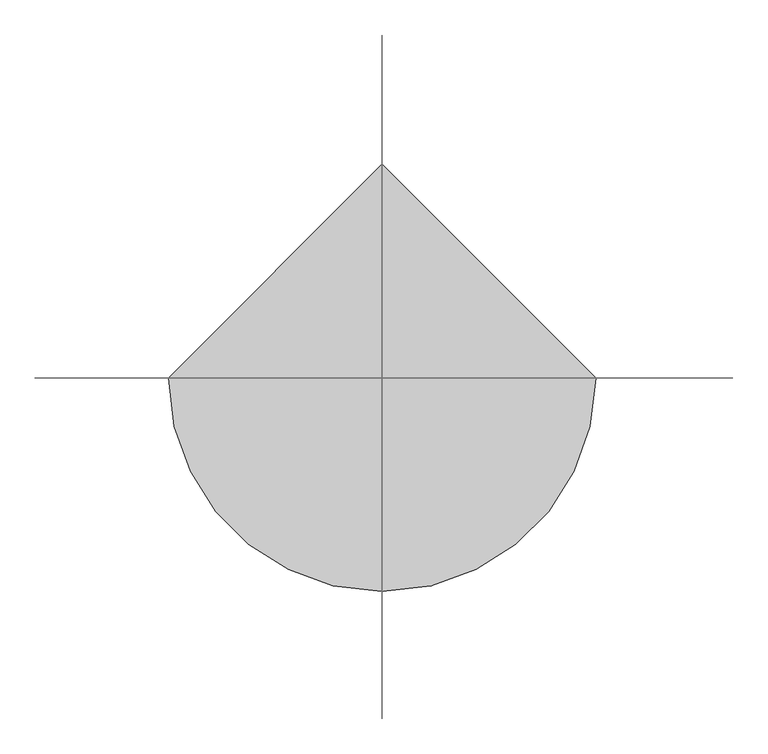
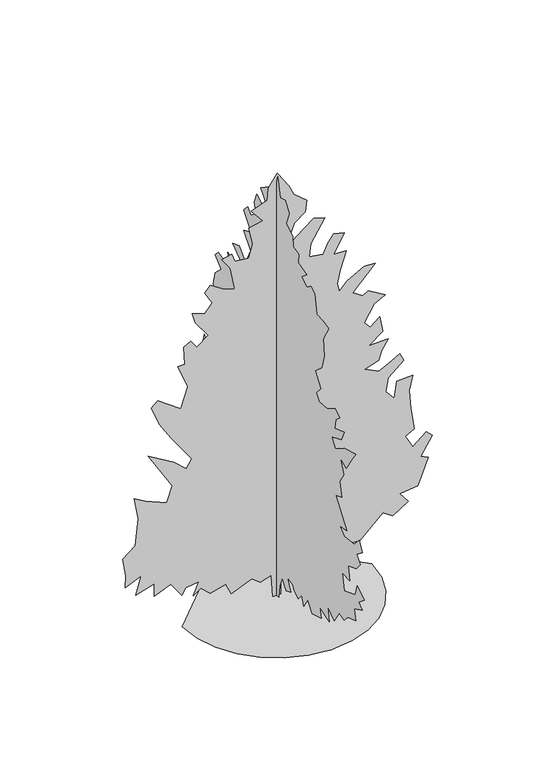
"""IFC4 building model written with IfcOpenShell, lengths in millimetres: proxy geometry, holly miniature 26078 : holly miniature 26078."""

import ifcopenshell
import ifcopenshell.guid

model = None  # the IFC model being written
_history = None  # IfcOwnerHistory: only IFC2X3 demands one
_inside = {}  # id of a spatial element -> (the spatial element, [elements in it])
_under = {}  # id of a project, library or spatial element -> (it, [spatial elements below it])
_declared = {}  # id of a project -> (the project, [libraries it declares])
_typed = {}  # id of a type object -> (the type object, [elements of that type])
_made_of = {}  # id of a material, layer set ... -> (it, [elements and type objects made of it])


def new_model(schema):
    """Start an empty IFC model of exactly this schema.

    Asked for "IFC4X3", IfcOpenShell would pick the latest addendum, in which some entities
    have other attributes; the version numbers below select the first issue.
    IFC2X3 requires an IfcOwnerHistory on every rooted entity: one is made here for all.
    """
    global model, _history
    if schema == "IFC4X3":
        model = ifcopenshell.file(schema_version=(4, 3, 0, 0))
    else:
        model = ifcopenshell.file(schema=schema)
    _inside.clear()
    _under.clear()
    _declared.clear()
    _typed.clear()
    _made_of.clear()
    _history = None
    if model.schema == "IFC2X3":
        org = make("IfcOrganization", Name="unknown")
        user = make(
            "IfcPersonAndOrganization",
            ThePerson=make("IfcPerson", FamilyName="unknown"),
            TheOrganization=org,
        )
        app = make(
            "IfcApplication",
            ApplicationDeveloper=org,
            Version="unknown",
            ApplicationFullName="unknown",
            ApplicationIdentifier="unknown",
        )
        _history = make(
            "IfcOwnerHistory",
            OwningUser=user,
            OwningApplication=app,
            ChangeAction="ADDED",
            CreationDate=0,
        )
    return model


def make(cls, **values):
    """One entity of the class cls with the attributes given. An attribute that is None is left unset."""
    return model.create_entity(
        cls, **{name: value for name, value in values.items() if value is not None}
    )


def rooted(cls, **values):
    """An entity with a GlobalId (a new one), such as an element, a storey or a relation."""
    return make(cls, GlobalId=ifcopenshell.guid.new(), OwnerHistory=_history, **values)


def si_unit(unit_type, name, prefix=None):
    """IfcSIUnit, for example si_unit("LENGTHUNIT", "METRE", prefix="MILLI")."""
    return make("IfcSIUnit", UnitType=unit_type, Prefix=prefix, Name=name)


def assignment(units):
    """IfcUnitAssignment: the units of a project."""
    return None if units is None else make("IfcUnitAssignment", Units=units)


def point(xyz):
    """IfcCartesianPoint."""
    return None if xyz is None else make("IfcCartesianPoint", Coordinates=xyz)


def direction(xyz):
    """IfcDirection."""
    return None if xyz is None else make("IfcDirection", DirectionRatios=xyz)


def frame(location, z_axis=None, x_axis=None):
    """IfcAxis2Placement3D, a coordinate frame: its origin and axes. An axis left out is left unset."""
    return make(
        "IfcAxis2Placement3D",
        Location=point(location),
        Axis=direction(z_axis),
        RefDirection=direction(x_axis),
    )


def origin():
    """The frame at (0, 0, 0) with its axes left unset."""
    return frame((0.0, 0.0, 0.0))


def place(relative_to, where):
    """IfcLocalPlacement: puts the frame where relative to a parent placement (None: the world)."""
    return make(
        "IfcLocalPlacement", PlacementRelTo=relative_to, RelativePlacement=where
    )


def context(
    kind, dimensions, precision=None, world=None, true_north=None, identifier=None
):
    """IfcGeometricRepresentationContext, for example the 3D "Model" context."""
    return make(
        "IfcGeometricRepresentationContext",
        ContextIdentifier=identifier,
        ContextType=kind,
        CoordinateSpaceDimension=dimensions,
        Precision=precision,
        WorldCoordinateSystem=world,
        TrueNorth=true_north,
    )


def project(units=None, contexts=None):
    """IfcProject with its units and contexts."""
    return rooted(
        "IfcProject",
        Name="project",
        RepresentationContexts=contexts,
        UnitsInContext=assignment(units),
    )


def spatial(cls, under=None, at=None, **own):
    """A site, building, storey or space (cls), placed at a placement, below another one or the project."""
    s = rooted(cls, ObjectPlacement=at, **own)
    if under is not None:
        _under.setdefault(under.id(), (under, []))[1].append(s)
    return s


def point_list(points):
    """IfcCartesianPointList2D or 3D."""
    cls = (
        "IfcCartesianPointList2D" if len(points[0]) == 2 else "IfcCartesianPointList3D"
    )
    return make(cls, CoordList=points)


def triangles(points, corners, closed=None, point_numbers=None):
    """IfcTriangulatedFaceSet: each triangle names its three corners, points numbered from 1."""
    return make(
        "IfcTriangulatedFaceSet",
        Coordinates=point_list(points),
        Closed=closed,
        CoordIndex=corners,
        PnIndex=point_numbers,
    )


def shape(context_of_items, identifier, shape_type, items):
    """IfcShapeRepresentation: the items that make up one representation, for example the "Body"."""
    return make(
        "IfcShapeRepresentation",
        ContextOfItems=context_of_items,
        RepresentationIdentifier=identifier,
        RepresentationType=shape_type,
        Items=items,
    )


def source(mapping_origin, context_of_items, identifier, shape_type, items):
    """IfcRepresentationMap: a shape defined once, which mapped items show again and again."""
    return make(
        "IfcRepresentationMap",
        MappingOrigin=mapping_origin,
        MappedRepresentation=shape(context_of_items, identifier, shape_type, items),
    )


def transform(
    local_origin,
    x_axis=None,
    y_axis=None,
    z_axis=None,
    scale=None,
    scale2=None,
    scale3=None,
    uniform=True,
):
    """IfcCartesianTransformationOperator3D, or its non-uniform kind. x_axis, y_axis, z_axis: its Axis1, 2, 3."""
    if uniform:
        return make(
            "IfcCartesianTransformationOperator3D",
            Axis1=direction(x_axis),
            Axis2=direction(y_axis),
            LocalOrigin=point(local_origin),
            Scale=scale,
            Axis3=direction(z_axis),
        )
    return make(
        "IfcCartesianTransformationOperator3DnonUniform",
        Axis1=direction(x_axis),
        Axis2=direction(y_axis),
        LocalOrigin=point(local_origin),
        Scale=scale,
        Axis3=direction(z_axis),
        Scale2=scale2,
        Scale3=scale3,
    )


def mapped(mapping_source, mapping_target):
    """IfcMappedItem: shows the shape of a source again, moved by a transform."""
    return make(
        "IfcMappedItem", MappingSource=mapping_source, MappingTarget=mapping_target
    )


def made_of(thing, what):
    """Note that an element or type object is made of a material, layer set ...; save() writes the relation."""
    if what is not None:
        _made_of.setdefault(what.id(), (what, []))[1].append(thing)
    return thing


def element(
    cls,
    number,
    at=None,
    inside=None,
    cuts=None,
    type_object=None,
    material=None,
    context=None,
    identifier="Body",
    shape_type=None,
    held_by="IfcProductDefinitionShape",
    body=None,
    shapes=None,
    **own,
):
    """One element of the class cls, such as IfcWall. Its Tag is "e" and its number.

    at: its placement. inside: the storey or other place that contains it. cuts: it is an
    opening in that element (IfcRelVoidsElement). A single representation is given by context,
    identifier, shape_type and body (its items); several are given by shapes. held_by: the class
    of the entity that holds the representations. save() writes the other relations.
    """
    e = rooted(cls, Tag="e%d" % number, ObjectPlacement=at, **own)
    if body is not None:
        shapes = [shape(context, identifier, shape_type, body)]
    if shapes is not None:
        e.Representation = make(held_by, Representations=shapes)
    if inside is not None:
        _inside.setdefault(inside.id(), (inside, []))[1].append(e)
    if cuts is not None:
        rooted(
            "IfcRelVoidsElement", RelatingBuildingElement=cuts, RelatedOpeningElement=e
        )
    if type_object is not None:
        _typed.setdefault(type_object.id(), (type_object, []))[1].append(e)
    return made_of(e, material)


def aggregate(whole, parts):
    """IfcRelAggregates: a whole, such as a stair, and the parts it consists of."""
    return rooted("IfcRelAggregates", RelatingObject=whole, RelatedObjects=parts)


def save(model, path):
    """Write the relations noted so far, then the file.

    IfcRelAggregates (storeys below a building ...), IfcRelContainedInSpatialStructure (elements
    in a storey), IfcRelDefinesByType, IfcRelAssociatesMaterial and IfcRelDeclares: one each for
    every whole, place, type object, material and project.
    """
    for whole, parts in _under.values():
        aggregate(whole, parts)
    for where, things in _inside.values():
        rooted(
            "IfcRelContainedInSpatialStructure",
            RelatedElements=things,
            RelatingStructure=where,
        )
    for kind, things in _typed.values():
        rooted("IfcRelDefinesByType", RelatedObjects=things, RelatingType=kind)
    for what, things in _made_of.values():
        rooted("IfcRelAssociatesMaterial", RelatedObjects=things, RelatingMaterial=what)
    for by, libraries in _declared.values():
        rooted("IfcRelDeclares", RelatingContext=by, RelatedDefinitions=libraries)
    model.write(path)


def entourage_9c913b6c(model_context):
    return source(origin(), model_context, "Body", "Tessellation", [
        triangles([(6e-07, 14.2176358, 1.67e-05), (3.9e-06, 26.9638997, 91.3171369), (5.3e-06, 55.4926929, 95.2500727), (6.3e-06, 99.9429821, 60.3250469), (1.03e-05, 160.2677792, 104.7750818), (1.07e-05, 192.0178034, 69.850056), (1.31e-05, 220.9545183, 106.6026137), (1.54e-05, 277.7441478, 101.6000848), (1.65e-05, 277.7441478, 136.525106), (2.16e-05, 376.1666831, 161.9251272), (3.77e-05, 611.119384, 349.2502665), (4.08e-05, 623.8168648, 431.8003512), (3.82e-05, 538.0918284, 476.2503633), (3.59e-05, 468.2417679, 501.6504118), (4.11e-05, 522.21678, 596.9004845), (4.62e-05, 588.8918527, 666.7505087), (4.6e-05, 534.9168042, 739.7755571), (4.75e-05, 515.8668042, 819.150654), (4.39e-05, 468.2417679, 771.5255814), (4.05e-05, 395.2166831, 765.1756056), (4.39e-05, 433.3167194, 822.3256783), (4.03e-05, 338.0691902, 844.5507025), (4.63e-05, 385.6916831, 974.7257509), (5.23e-05, 452.3667558, 1076.325872), (5.33e-05, 436.4917437, 1133.475872), (5.27e-05, 395.2166831, 1174.7509689), (5.57e-05, 436.4917437, 1212.8509689), (5.55e-05, 417.4442508, 1235.0759205), (5.08e-05, 328.5416468, 1212.8509689), (5.36e-05, 347.5916468, 1276.3510174), (4.79e-05, 255.5191236, 1222.3759689), (4.96e-05, 249.1678579, 1289.0509689), (5.38e-05, 312.6666347, 1336.6761143), (5.23e-05, 268.2165862, 1352.5510174), (4.99e-05, 236.4678337, 1320.8010658), (4.67e-05, 188.8427974, 1282.7010658), (4.91e-05, 204.7178095, 1339.8510658), (4.95e-05, 185.6677913, 1381.1261627), (5.34e-05, 233.2928277, 1441.4511143), (5.18e-05, 182.4928034, 1463.6762112), (5.6e-05, 233.2928277, 1530.3512112), (5.58e-05, 207.8928155, 1558.9262112), (5.41e-05, 185.6677913, 1536.7012596), (5.33e-05, 147.5677641, 1568.4512112), (5.5e-05, 160.2677792, 1606.5513565), (5.56e-05, 141.217761, 1654.1763565), (5.22e-05, 87.2427217, 1619.2513081), (5.18e-05, 65.017702, 1641.4762596), (5.57e-05, 112.6427429, 1698.626405), (5.41e-05, 49.1426899, 1743.0764534), (5.31e-05, 7.8675799, 1768.4763565), (5.39e-05, -8.0073817, 1819.2764534), (5.08e-05, -22.8780526, 1737.2217236), (4.95e-05, -58.8071436, 1749.4263565), (4.7e-05, -87.3824206, 1708.151405), (4.62e-05, -68.3324025, 1654.1763565), (4.34e-05, -112.7824418, 1625.6013565), (4.19e-05, -115.9574388, 1581.1513081), (3.99e-05, -157.2324812, 1574.8012596), (3.9e-05, -150.8824691, 1533.5261627), (3.58e-05, -211.2075115, 1517.6512596), (3.65e-05, -176.2824994, 1489.0762596), (3.42e-05, -211.2075115, 1463.6762112), (3.36e-05, -239.7825478, 1485.9011627), (3.18e-05, -271.5338438, 1473.2012112), (2.87e-05, -284.2338498, 1390.6511627), (2.66e-05, -331.8588861, 1390.6511627), (2.46e-05, -369.9589225, 1381.1261627), (2.43e-05, -331.8588861, 1314.4510174), (2.19e-05, -338.2088983, 1241.4259689), (2.09e-05, -319.1588619, 1181.1009447), (2.17e-05, -274.7088316, 1139.8259205), (1.84e-05, -312.8088861, 1085.850872), (1.87e-05, -281.0588438, 1047.750872), (1.69e-05, -303.283868, 1022.3508236), (1.46e-05, -357.6551313, 1025.5435793), (1.31e-05, -414.4089346, 1060.4508236), (1.11e-05, -446.1589588, 1041.4008236), (1.15e-05, -420.7589467, 1016.0008478), (1.07e-05, -411.2314033, 974.7257509), (8.3e-06, -477.9090194, 996.9507751), (7.9e-06, -458.858983, 952.5007267), (1.01e-05, -389.0089225, 923.9257267), (7.9e-06, -415.6357856, 888.360601), (6.2e-06, -481.0840073, 930.2757751), (3.3e-06, -560.4590678, 952.5007267), (3.4e-06, -531.8840315, 911.2257025), (3.3e-06, -493.7840315, 850.9006783), (5.8e-06, -449.333983, 869.9506783), (2.9e-06, -477.0326921, 812.787961), (2.9e-06, -446.1564517, 765.1756056), (4e-07, -462.0340073, 704.8505814), (1.7e-06, -420.7589467, 688.9755329), (-4.9e-06, -496.9564759, 581.0254724), (-2.9e-06, -446.1564517, 571.5004724), (-5.1e-06, -477.9090194, 546.1004239), (-8.1e-06, -550.9340678, 555.6254602), (-8.5e-06, -585.8590799, 593.7254602), (-1.07e-05, -608.0841042, 552.450436), (-9.8e-06, -566.8090799, 520.7004118), (-1.18e-05, -592.209092, 492.1254118), (-1.16e-05, -563.6340557, 457.2003633), (-9.7e-06, -506.4840194, 434.9753391), (-1.19e-05, -519.1840436, 377.8253028), (-9.5e-06, -465.8973252, 379.8446199), (-1.22e-05, -481.0814638, 311.1502665), (-1.48e-05, -557.2840799, 339.7252665), (-1.39e-05, -569.9840678, 387.3503028), (-1.72e-05, -620.7841284, 355.6002786), (-1.64e-05, -582.684092, 323.8502543), (-1.81e-05, -608.0841042, 304.8002543), (-1.64e-05, -550.9340678, 276.225218), (-1.82e-05, -560.4590678, 228.6001817), (-1.63e-05, -503.306488, 209.5501635), (-1.6e-05, -477.9090194, 180.9751453), (-1.41e-05, -442.9839709, 190.5001453), (-1.42e-05, -408.0564154, 136.525106), (-1.11e-05, -360.4339225, 168.2751393), (-1.34e-05, -373.1313669, 111.1250848), (-9.7e-06, -306.458874, 133.350109), (-1.14e-05, -315.9813306, 92.0750757), (-9.1e-06, -252.4825539, 73.0250575), (-6.5e-06, -220.7325296, 114.3000908), (-6.5e-06, -192.1575115, 69.850056), (-4.7e-06, -176.2824994, 107.9500878), (-4.5e-06, -150.8824691, 76.2000636), (-2.8e-06, -125.4824479, 95.2500727), (-1.6e-06, -112.7824418, 114.3000908), (4e-07, -74.68241, 123.8250999), (-2.3e-06, -100.0824267, 73.0250575), (-1.3e-06, -68.3324025, 60.3250469), (1.2e-06, -39.7573798, 98.4250787), (7e-07, -20.0124481, 53.1848487), (-6e-07, -14.3573869, 1.58e-05), (-16.1742762, 3.5e-06, 1.68e-05), (-22.5242565, -5e-07, 95.2500727), (-66.9742641, 1.5e-06, 79.3750606), (-101.8992944, 1.2e-06, 107.9500878), (-187.6243579, 5.4e-06, 73.0250575), (-209.8493822, 3.9e-06, 120.6500939), (-273.3499393, 6.5e-06, 104.7750818), (-311.4499575, 6.1e-06, 139.700112), (-343.1999817, 8e-06, 117.4750969), (-320.9749938, 4.9e-06, 171.4501453), (-372.9815214, 6.8e-06, 163.8728099), (-390.825018, 8.6e-06, 136.525106), (-435.2750665, 7.1e-06, 200.0251635), (-501.9501391, 1.71e-05, 171.4501453), (-501.9501391, 7.9e-06, 225.4251756), (-578.1501755, 1.8e-05, 203.2001696), (-555.9251513, 7.1e-06, 279.4002241), (-622.6002239, 1.72e-05, 250.8252059), (-619.4251997, 1.48e-05, 301.6252483), (-632.1252239, 5e-06, 377.8253028), (-581.3251997, 1.6e-06, 419.100327), (-568.6251755, -3.7e-06, 530.2254118), (-584.5001876, -7.4e-06, 622.3005329), (-540.0501391, -7.6e-06, 596.9004845), (-451.1500786, -8.5e-06, 558.8004481), (-428.9250544, -1.9e-05, 625.4754845), (-492.4251028, -2.17e-05, 730.2505571), (-527.3501513, -2.33e-05, 787.4006298), (-422.5750422, -2.35e-05, 723.9005814), (-371.775018, -2.31e-05, 679.4505329), (-349.5499938, -2.53e-05, 714.3755814), (-432.1000786, -2.81e-05, 831.8506783), (-482.9001028, -3.01e-05, 911.2257025), (-514.650127, -3.27e-05, 990.6007994), (-489.2501149, -3.46e-05, 1016.0008478), (-394.0000422, -3.43e-05, 946.1507509), (-365.4250059, -4.58e-05, 1031.8758236), (-406.7000301, -4.91e-05, 1133.475872), (-378.1250301, -5e-05, 1133.475872), (-381.300018, -5.33e-05, 1209.6759447), (-352.725018, -5.49e-05, 1225.5509205), (-327.3249696, -5.41e-05, 1190.6259447), (-280.5940284, -5.71e-05, 1227.0368763), (-333.6749817, -5.87e-05, 1298.5759689), (-346.3750059, -6.03e-05, 1343.0260174), (-295.5749635, -6.1e-05, 1323.9760174), (-263.8249393, -6.36e-05, 1362.0760174), (-295.1355281, -7.18e-05, 1414.3061142), (-273.2864439, -7.37e-05, 1441.3724854), (-216.1993761, -7.37e-05, 1403.3511143), (-171.7493458, -7.44e-05, 1390.6511627), (-190.799364, -7.81e-05, 1485.9011627), (-225.7243943, -7.92e-05, 1533.5261627), (-183.7899808, -8.09e-05, 1543.2950432), (-171.7493458, -7.97e-05, 1508.1262596), (-114.5993004, -8.11e-05, 1501.7762112), (-98.7242883, -8.41e-05, 1558.9262112), (-114.5993004, -8.69e-05, 1631.9512596), (-57.4492595, -9.6e-05, 1644.6513565), (-105.0743004, -9.72e-05, 1701.8013565), (-38.3992414, -0.0001003, 1727.201405), (-35.2242399, -0.0001026, 1778.0013565), (2.8758411, -0.0001061, 1828.8014534), (48.9753037, -0.0001044, 1760.0893684), (69.5505876, -0.0001029, 1714.5013081), (123.5258904, -0.0001026, 1670.051405), (117.1758782, -0.0001002, 1622.4262596), (71.0844965, -9.73e-05, 1587.6612305), (28.2758109, -8.41e-05, 1473.2012112), (79.075851, -9.48e-05, 1527.1762596), (152.1009085, -9.94e-05, 1581.1513081), (196.5509388, -0.0001002, 1568.4512112), (139.4009025, -9.44e-05, 1476.3761627), (133.0508904, -8.5e-05, 1422.4011143), (190.2009449, -9.3e-05, 1412.8761143), (209.250963, -9.55e-05, 1454.1512112), (234.6509751, -9.76e-05, 1485.9011627), (275.9255088, -9.84e-05, 1476.3761627), (234.6509751, -9.37e-05, 1397.0010658), (285.4505088, -9.5e-05, 1393.8261143), (260.0504967, -8.42e-05, 1320.8010658), (247.3509812, -8.13e-05, 1263.6510658), (256.8754907, -8e-05, 1228.7260174), (288.6255149, -8.25e-05, 1263.6510658), (358.4755754, -9.31e-05, 1301.7510658), (402.9255876, -9.43e-05, 1298.5759689), (310.8505391, -8.05e-05, 1203.3259689), (352.1255633, -8.04e-05, 1174.7509689), (374.3505876, -8.18e-05, 1190.6259447), (445.2877547, -8.2e-05, 1148.1927063), (399.7505997, -7.96e-05, 1123.950872), (358.4755754, -7.53e-05, 1057.275872), (383.8755876, -7.48e-05, 1028.7007994), (421.9756239, -7.74e-05, 1060.4508236), (434.6756118, -7.48e-05, 993.7758236), (377.5255754, -7.11e-05, 949.3257751), (456.900636, -7.36e-05, 952.5007267), (431.5006239, -7.1e-05, 911.2257025), (418.8005997, -6.89e-05, 873.1257025), (361.6505633, -6.64e-05, 854.0757025), (418.8005997, -6.68e-05, 825.5006298), (457.6550231, -6.87e-05, 843.1206299), (504.5256723, -7.13e-05, 869.9506783), (520.4006845, -7.04e-05, 838.200654), (456.900636, -6.61e-05, 784.2256056), (447.375636, -6.32e-05, 727.0756056), (482.3006481, -6.24e-05, 685.8005814), (491.8256845, -6.58e-05, 755.6506056), (558.5007208, -6.8e-05, 758.8256298), (542.6257087, -6.48e-05, 698.5005329), (548.9757208, -6.14e-05, 619.1255087), (564.8507329, -5.08e-05, 523.875436), (526.7506966, -4.89e-05, 504.8253997), (558.5007208, -4.72e-05, 447.6753633), (612.4757692, -5.1e-05, 495.3003997), (637.8758177, -5.06e-05, 469.9003876), (590.250745, -4.59e-05, 396.8753028), (622.0007692, -4.62e-05, 381.0002907), (577.5507571, -4e-05, 273.050212), (504.5256723, -3.74e-05, 263.525212), (539.4507208, -3.65e-05, 219.0751817), (475.9506723, -2.59e-05, 177.8001393), (434.6756118, -2.6e-05, 206.3751575), (339.4255391, -1.91e-05, 117.4750969), (291.8005209, -1.79e-05, 120.6500939), (215.600957, -1.33e-05, 69.850056), (164.8009146, -1.38e-05, 114.3000908), (120.3508843, -4e-06, 76.2000636), (88.6008601, -3.7e-06, 92.0750757), (47.3258268, -4e-07, 44.4500348), (18.7507268, -2.3e-06, 107.9500878), (15.5757242, 2.6e-06, 1.58e-05), (-388.6203197, 1e-06, 2.79e-05), (-378.3460196, -89.0461181, 2.49e-05), (-349.0877037, -170.8207325, 2.16e-05), (-303.1848006, -242.9809173, 1.81e-05), (-242.9809173, -303.1848006, 1.45e-05), (-170.8207325, -349.0877037, 1.1e-05), (-89.0461181, -378.3460196, 7.7e-06), (1.7e-05, -388.6203197, 4.7e-06), (89.0461181, -378.3460196, 2.3e-06), (170.8207325, -349.0877037, 8e-07), (242.9809173, -303.1848006, 0.0), (303.1848006, -242.9809173, 0.0), (349.0877037, -170.8207325, 8e-07), (378.3460196, -89.0461181, 2.3e-06), (388.6203197, 3.91e-05, 4.7e-06), (-5.1e-05, 388.6203197, 2.79e-05)], [[51, 52, 53], [85, 86, 87], [29, 30, 31], [80, 81, 82], [80, 82, 83], [60, 61, 62], [123, 124, 125], [32, 33, 34], [32, 34, 35], [17, 18, 19], [118, 119, 120], [110, 111, 112], [93, 94, 95], [20, 21, 22], [97, 98, 99], [97, 99, 100], [108, 109, 110], [107, 108, 110], [32, 35, 36], [67, 68, 69], [103, 104, 105], [38, 39, 40], [77, 78, 79], [76, 77, 79], [85, 87, 88], [85, 88, 89], [84, 85, 89], [45, 46, 47], [5, 6, 7], [44, 45, 47], [7, 8, 9], [48, 49, 50], [129, 130, 131], [129, 131, 132], [76, 79, 80], [41, 42, 43], [40, 41, 43], [107, 110, 112], [106, 107, 112], [116, 117, 118], [31, 32, 36], [58, 59, 60], [66, 67, 69], [125, 126, 127], [26, 27, 28], [26, 28, 29], [120, 121, 122], [120, 122, 123], [133, 134, 1], [133, 1, 2], [132, 133, 2], [91, 92, 93], [112, 113, 114], [106, 112, 114], [100, 101, 102], [15, 16, 17], [50, 51, 53], [48, 50, 53], [72, 73, 74], [3, 4, 5], [53, 54, 55], [53, 55, 56], [48, 53, 56], [96, 97, 100], [96, 100, 102], [96, 102, 103], [11, 12, 13], [10, 11, 13], [10, 13, 14], [125, 127, 128], [76, 80, 83], [75, 76, 83], [15, 17, 19], [15, 19, 20], [14, 15, 20], [114, 115, 116], [106, 114, 116], [9, 10, 14], [63, 64, 65], [63, 65, 66], [89, 90, 91], [84, 89, 91], [106, 116, 118], [56, 57, 58], [48, 56, 58], [47, 48, 58], [40, 43, 44], [105, 106, 118], [96, 103, 105], [95, 96, 105], [44, 47, 58], [40, 44, 58], [40, 58, 60], [38, 40, 60], [38, 60, 62], [38, 62, 63], [38, 63, 66], [37, 38, 66], [36, 37, 66], [36, 66, 69], [36, 69, 70], [36, 70, 71], [36, 71, 72], [36, 72, 74], [31, 36, 74], [23, 24, 25], [23, 25, 26], [23, 26, 29], [23, 29, 31], [23, 31, 74], [22, 23, 74], [22, 74, 75], [22, 75, 83], [22, 83, 84], [22, 84, 91], [22, 91, 93], [22, 93, 95], [20, 22, 95], [14, 20, 95], [9, 14, 95], [7, 9, 95], [5, 7, 95], [3, 5, 95], [2, 3, 95], [132, 2, 95], [129, 132, 95], [129, 95, 105], [129, 105, 118], [128, 129, 118], [125, 128, 118], [123, 125, 118], [120, 123, 118], [161, 162, 163], [142, 143, 144], [219, 220, 221], [218, 219, 221], [156, 157, 158], [178, 179, 180], [160, 161, 163], [160, 163, 164], [230, 231, 232], [149, 150, 151], [223, 224, 225], [227, 228, 229], [217, 218, 221], [151, 152, 153], [263, 264, 265], [147, 148, 149], [186, 187, 188], [186, 188, 189], [171, 172, 173], [145, 146, 147], [196, 197, 198], [193, 194, 195], [227, 229, 230], [242, 243, 244], [241, 242, 244], [205, 206, 207], [204, 205, 207], [213, 214, 215], [222, 223, 225], [211, 212, 213], [210, 211, 213], [209, 210, 213], [195, 196, 198], [241, 244, 245], [254, 255, 256], [254, 256, 257], [236, 237, 238], [236, 238, 239], [235, 236, 239], [177, 178, 180], [156, 158, 159], [191, 192, 193], [265, 266, 135], [265, 135, 136], [138, 139, 140], [203, 204, 207], [203, 207, 208], [248, 249, 250], [248, 250, 251], [195, 198, 199], [251, 252, 253], [182, 183, 184], [181, 182, 184], [193, 195, 199], [174, 175, 176], [173, 174, 176], [168, 169, 170], [167, 168, 170], [166, 167, 170], [251, 253, 254], [222, 225, 226], [259, 260, 261], [230, 232, 233], [230, 233, 234], [245, 246, 247], [155, 156, 159], [193, 199, 200], [193, 200, 201], [193, 201, 202], [191, 193, 202], [191, 202, 203], [190, 191, 203], [261, 262, 263], [248, 251, 254], [151, 153, 154], [151, 154, 155], [136, 137, 138], [181, 184, 185], [140, 141, 142], [140, 142, 144], [241, 245, 247], [186, 189, 190], [185, 186, 190], [185, 190, 203], [165, 166, 170], [151, 155, 159], [149, 151, 159], [147, 149, 159], [145, 147, 159], [144, 145, 159], [221, 222, 226], [235, 239, 240], [209, 213, 215], [209, 215, 216], [208, 209, 216], [171, 173, 176], [177, 180, 181], [177, 181, 185], [185, 203, 208], [185, 208, 216], [177, 185, 216], [177, 216, 217], [234, 235, 240], [140, 144, 159], [138, 140, 159], [138, 159, 160], [138, 160, 164], [138, 164, 165], [136, 138, 165], [265, 136, 165], [257, 258, 259], [217, 221, 226], [177, 217, 226], [176, 177, 226], [171, 176, 226], [170, 171, 226], [165, 170, 226], [265, 165, 226], [265, 226, 227], [265, 227, 230], [265, 230, 234], [265, 234, 240], [263, 265, 240], [261, 263, 240], [259, 261, 240], [257, 259, 240], [257, 240, 241], [257, 241, 247], [254, 257, 247], [248, 254, 247], [281, 282, 267], [280, 281, 267], [280, 267, 268], [279, 280, 268], [279, 268, 269], [279, 269, 270], [278, 279, 270], [277, 278, 270], [277, 270, 271], [277, 271, 272], [277, 272, 273], [277, 273, 274], [277, 274, 275], [277, 275, 276]], closed=False),
    ])


if __name__ == "__main__":
    model = new_model("IFC4")
    model_context = context("Model", 3, world=origin())
    ifc_project = project(units=[si_unit("LENGTHUNIT", "METRE", prefix="MILLI")], contexts=[model_context])
    site = spatial("IfcSite", under=ifc_project)
    building = spatial("IfcBuilding", under=site)
    placement = place(None, origin())
    entourage_shape = entourage_9c913b6c(model_context)
    element("IfcBuildingElementProxy", 1, Name="holly miniature 26078 : holly miniature 26078", ObjectType="holly miniature 26078 : holly miniature 26078", at=placement, inside=building, context=model_context, shape_type="MappedRepresentation", body=[
        mapped(entourage_shape, transform((0.0, 0.0, 0.0), x_axis=(1.0, 0.0, 0.0), y_axis=(0.0, 1.0, 0.0), z_axis=(0.0, 0.0, 1.0))),
    ])
    save(model, "model.ifc")

# Revit data of these elements
# Type "holly miniature 26078 : holly miniature 26078"
#   built-in parameter 1005195 = "RPC-16-FXGU-6LXX-PKLL-J000-ST1L-LVER-AU"
#   Height = 0
